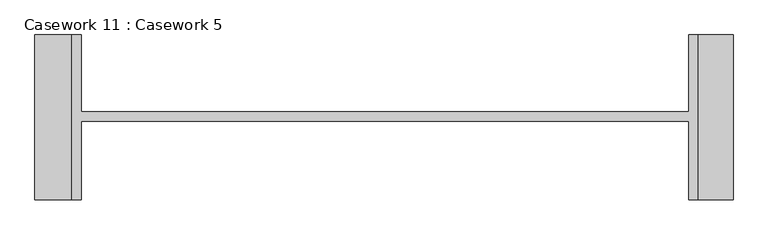
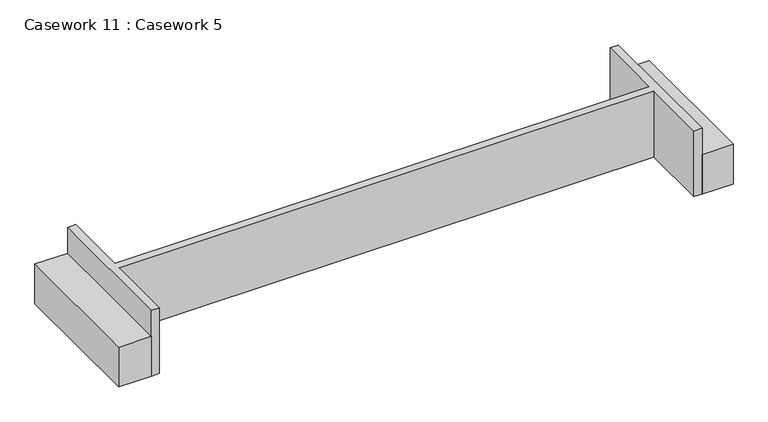
"""IFC4 building model written with IfcOpenShell, lengths in millimetres: furniture geometry, Casework 11 : Casework 5."""

from ifc_helpers import new_model, si_unit, origin, origin_with_axes, place, context, project, spatial, polyline, outline, extrude, source, transform, mapped, element, save


def casework_11_casework_5_22f72c83(model_context):
    return source(origin(), model_context, "Body", "SweptSolid", [
        extrude(outline(polyline([(-45222.23615, 268650.5344182), (-45222.23615, 266109.4831087), (-45765.6431786, 266109.4831087), (-45765.6431786, 268650.5344182), (-45222.23615, 268650.5344182)])), origin_with_axes(), (0.0, 0.0, 1.0), 736.6),
        extrude(outline(polyline([(-55407.3218514, 268650.5344182), (-55407.3218514, 266109.4831087), (-55978.0010565, 266109.4831087), (-55978.0010565, 268650.5344182), (-55407.3218514, 268650.5344182)])), origin_with_axes(), (0.0, 0.0, 1.0), 736.6),
        extrude(outline(polyline([(-55264.4443999, 268650.5344182), (-55264.4443999, 267463.3259038), (-45907.3606126, 267463.3259038), (-45907.3606126, 268650.5344182), (-45765.6431786, 268650.5344182), (-45765.6431786, 266109.4831087), (-45907.3606126, 266109.4831087), (-45907.3606126, 267321.4625853), (-55264.4443999, 267321.4625853), (-55264.4443999, 266109.4831087), (-55407.3218514, 266109.4831087), (-55407.3218514, 268650.5344182), (-55264.4443999, 268650.5344182)])), origin_with_axes(), (0.0, 0.0, 1.0), 1219.2),
    ])


if __name__ == "__main__":
    model = new_model("IFC4")
    model_context = context("Model", 3, world=origin())
    ifc_project = project(units=[si_unit("LENGTHUNIT", "METRE", prefix="MILLI")], contexts=[model_context])
    site = spatial("IfcSite", under=ifc_project)
    building = spatial("IfcBuilding", under=site)
    placement = place(None, origin())
    casework_11_casework_5_shape = casework_11_casework_5_22f72c83(model_context)
    element("IfcFurniture", 1, ObjectType="Casework 11 : Casework 5", at=placement, inside=building, context=model_context, shape_type="MappedRepresentation", body=[
        mapped(casework_11_casework_5_shape, transform((0.0, 0.0, 0.0), x_axis=(1.0, 0.0, 0.0), y_axis=(0.0, 1.0, 0.0), z_axis=(0.0, 0.0, 1.0))),
    ])
    save(model, "model.ifc")

# Revit data of these elements
# Element 1 (IfcFurniture, "Casework 11 : Casework 5")
#   Materials on its faces: "Casework-oakfire"
# Materials
#   "Casework-oakfire": class "Miscellaneous", colour RGB 164 164 164, transparency 0, Cost = 0
